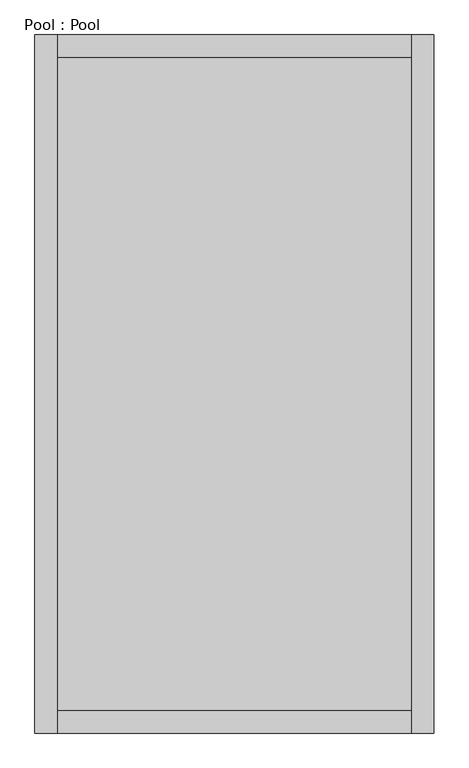
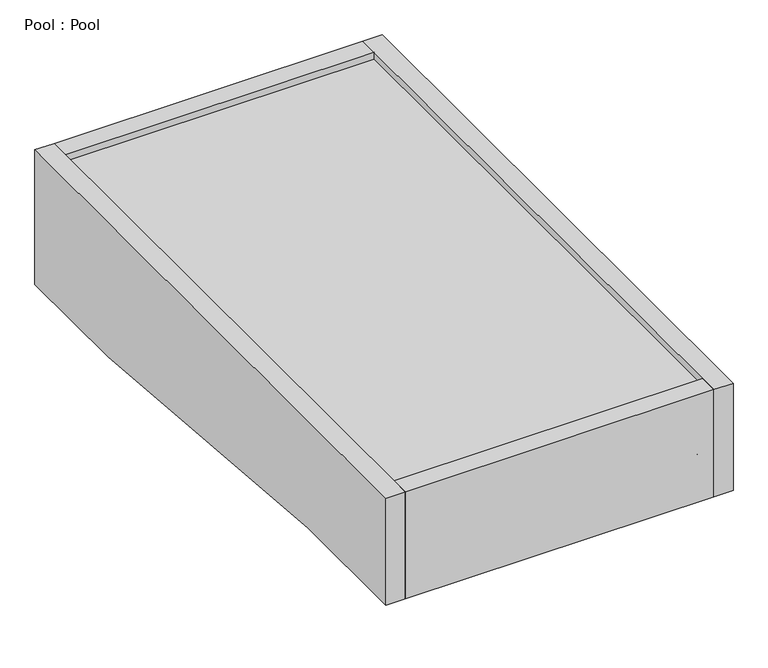
"""IFC4 building model written with IfcOpenShell, lengths in millimetres: proxy geometry, Pool : Pool."""

from ifc_helpers import new_model, si_unit, point, frame, frame_2d, origin, place, context, project, spatial, polyline, circle_curve, trimmed, segment, composite_curve, outline, extrude, source, transform, mapped, element, save


def pool_pool_4eb2a78d(model_context):
    return source(origin(), model_context, "Body", "SweptSolid", [
        extrude(outline(polyline([(-3200.4, 0.0), (3200.4, 0.0), (3200.4, -1498.6), (1871.1479816, -1498.6), (-1786.4520184, -1193.8), (-3200.4, -1193.8), (-3200.4, 0.0)])), frame((3251.2, 0.0, 0.0), z_axis=(1.0, 0.0, 0.0), x_axis=(0.0, 1.0, 0.0)), (0.0, 0.0, 1.0), 203.2),
        extrude(outline(polyline([(-3200.4, 0.0), (3200.4, 0.0), (3200.4, -1498.6), (1871.1479816, -1498.6), (-1786.4520184, -1193.8), (-3200.4, -1193.8), (-3200.4, 0.0)])), frame((-203.2, 0.0, 0.0), z_axis=(1.0, 0.0, 0.0), x_axis=(0.0, 1.0, 0.0)), (0.0, 0.0, 1.0), 203.2),
        extrude(outline(composite_curve([segment(polyline([(3200.4, -1498.6), (1871.1479816, -1498.6), (-1786.4520184, -1193.8), (-3200.4, -1193.8), (-3200.4, 0.0), (-2997.2, 0.0), (-2997.2, -685.8)]), True, "CONTINUOUS"), segment(trimmed(circle_curve(frame_2d((-2692.4, -685.8)), 304.8), [point((-2997.2, -685.8))], [point((-2692.4, -990.6))], True, "CARTESIAN"), True, "CONTINUOUS"), segment(polyline([(-2692.4, -990.6), (-1778.0, -990.6), (1879.6, -1295.4), (2692.4, -1295.4)]), True, "CONTINUOUS"), segment(trimmed(circle_curve(frame_2d((2692.4, -990.6)), 304.8), [point((2692.4, -1295.4))], [point((2997.2, -990.6))], True, "CARTESIAN"), True, "CONTINUOUS"), segment(polyline([(2997.2, -990.6), (2997.2, 0.0), (3200.4, 0.0), (3200.4, -1498.6)]), True, "CONTINUOUS")], self_intersect=False)), frame((0.0, 0.0, 0.0), z_axis=(1.0, 0.0, 0.0), x_axis=(0.0, 1.0, 0.0)), (0.0, 0.0, 1.0), 3251.2),
        extrude(outline(composite_curve([segment(polyline([(-2997.2, -76.2), (2997.2, -76.2), (2997.2, -990.6)]), True, "CONTINUOUS"), segment(trimmed(circle_curve(frame_2d((2692.4, -990.6)), 304.8), [point((2997.2, -990.6))], [point((2692.4, -1295.4))], False, "CARTESIAN"), True, "CONTINUOUS"), segment(polyline([(2692.4, -1295.4), (1879.6, -1295.4), (-1778.0, -990.6), (-2692.4, -990.6)]), True, "CONTINUOUS"), segment(trimmed(circle_curve(frame_2d((-2692.4, -685.8)), 304.8), [point((-2692.4, -990.6))], [point((-2997.2, -685.8))], False, "CARTESIAN"), True, "CONTINUOUS"), segment(polyline([(-2997.2, -685.8), (-2997.2, -76.2)]), True, "CONTINUOUS")], self_intersect=False)), frame((0.0, 0.0, 0.0), z_axis=(1.0, 0.0, 0.0), x_axis=(0.0, 1.0, 0.0)), (0.0, 0.0, 1.0), 3251.2),
    ])


if __name__ == "__main__":
    model = new_model("IFC4")
    model_context = context("Model", 3, world=origin())
    ifc_project = project(units=[si_unit("LENGTHUNIT", "METRE", prefix="MILLI")], contexts=[model_context])
    site = spatial("IfcSite", under=ifc_project)
    building = spatial("IfcBuilding", under=site)
    placement = place(None, origin())
    pool_pool_shape = pool_pool_4eb2a78d(model_context)
    element("IfcBuildingElementProxy", 1, Name="Pool : Pool", ObjectType="Pool : Pool", at=placement, inside=building, context=model_context, shape_type="MappedRepresentation", body=[
        mapped(pool_pool_shape, transform((0.0, 0.0, 0.0), x_axis=(1.0, 0.0, 0.0), y_axis=(0.0, 1.0, 0.0), z_axis=(0.0, 0.0, 1.0))),
    ])
    save(model, "model.ifc")

# Revit data of these elements
# Element 1 (IfcBuildingElementProxy, "Pool : Pool")
#   Materials on its faces: "Glass"
# Materials
#   "Glass": class "Unassigned", colour RGB 0 0 255, transparency 0.75
